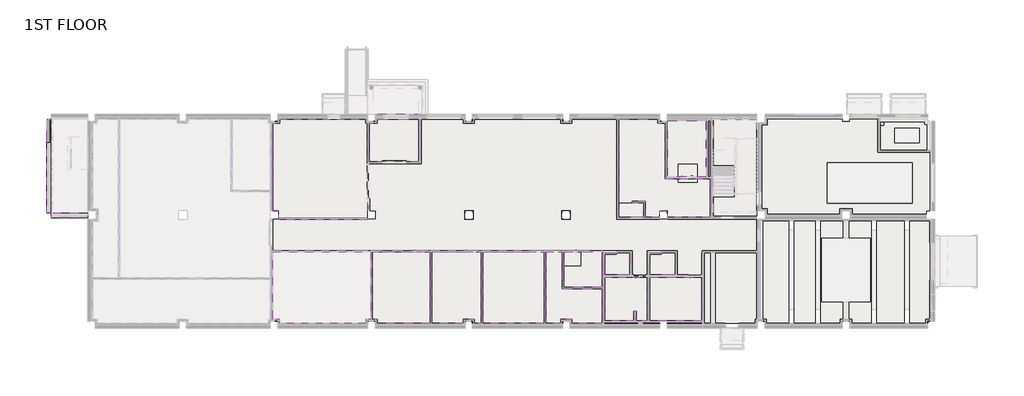
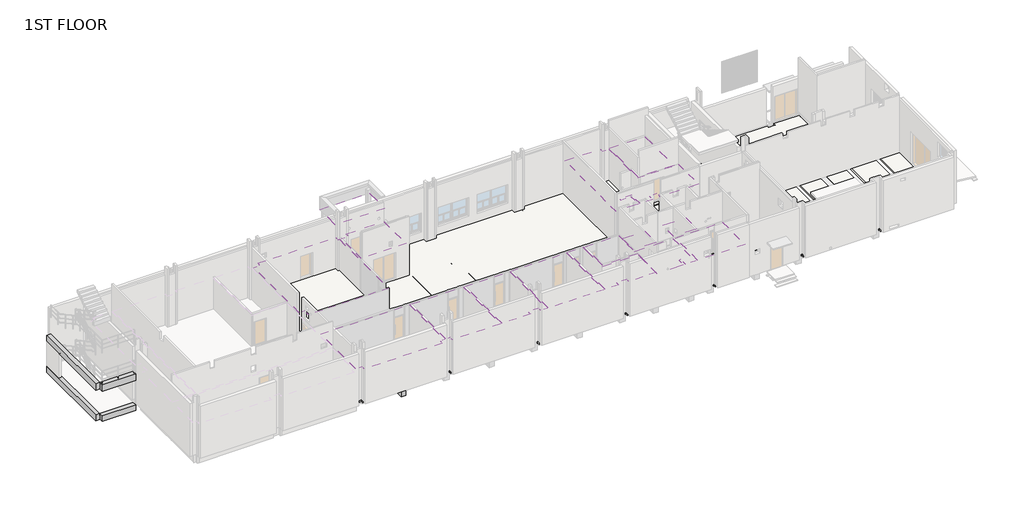
# One storey, part 8 of 15: 26 slabs, 15 coverings, 5 beams.
# Revit data of these elements (continued)
# Type "H_CE_AR_B09_2L Gypsum Board_T Bar_9T_C4" (continued)
#   Layers, outside or top first: 9.5 mm "00_Finish_Gypsum Board" (function 4); 9.5 mm "00_Finish_Gypsum Board" (function 4)
# Type "H_CE_AR_B09_Aluminum Spandrel_M Bar_0.8T_C9"
#   built-in parameter 1002203 = 1 (stored number, unit not read)
#   built-in parameter 1002202 = 1 (stored number, unit not read)
#   Layers, outside or top first: 0.8 mm "00.Ceiling_Aluminum Spandrel" (function 4)
# Type "H_CE_AR_B09_SMC Ceiling_T Bar_300x300x0.8T_C6"
#   built-in parameter 1002203 = 1 (stored number, unit not read)
#   built-in parameter 1002202 = 1 (stored number, unit not read)
#   Layers, outside or top first: 0.8 mm "00.Ceiling_SMC" (function 4)
# Type "H_CE_AR_B09_Souns Absorbing Soft Fiber Board_T Bar_600x600x9T_C5"
#   built-in parameter 1002203 = 1 (stored number, unit not read)
#   built-in parameter 1002202 = 1 (stored number, unit not read)
#   Layers, outside or top first: 9 mm "00.Ceiling_Sound Absorbing Soft Fiber Board" (function 4)
# Type "H_CE_AR_B09_Stainless Hairline Finish_3T"
#   built-in parameter 1002203 = 1 (stored number, unit not read)
#   built-in parameter 1002202 = 1 (stored number, unit not read)
#   Layers, outside or top first: 3 mm "00.Finish_Stainless Hairline" (function 4)
# Type "H_FL_AR_S17_RC Slab_T150_1S1"
#   Keynote = ""
#   Type Comments = "CV-AG"
#   Description = ""
#   H_Rebar Ratio = 0.1
#   Function = 1
#   Layers, outside or top first: 150 mm "Concrete_f'c=28MPa(Cylender)" (function 1)
# Type "H_FL_AR_S17_RC Slab_T150_GS1"
#   Keynote = ""
#   Type Comments = "CV-AG"
#   Description = ""
#   H_Rebar Ratio = 0.1
#   Function = 1
#   Layers, outside or top first: 150 mm "Concrete_f'c=28MPa(Cylender)" (function 1)
# Type "H_FL_AR_S17_RC Slab_T200_SS1"
#   Keynote = ""
#   Type Comments = "CV-AG"
#   Description = ""
#   H_Rebar Ratio = 0.1
#   Function = 1
#   Layers, outside or top first: 200 mm "Concrete_f'c=28MPa(Cylender)" (function 1)
# Type "H_FL_AR_B07_Wood Tile_600x600xT3_F8"
#   Keynote = ""
#   Type Comments = "Finish"
#   Description = ""
#   Function = 1
#   Layers, outside or top first: 3 mm "00_Finish_Wood Tile" (function 4); 27 mm "00_Concrete_Cement Mortar" (function 1)
# Type "H_FL_AR_B07_Deco Tile_600x600xT3"
#   Keynote = ""
#   Type Comments = "Finish"
#   Description = ""
#   Function = 1
#   Layers, outside or top first: 3 mm "00_Finish_Deco Tile" (function 4); 27 mm "00_Concrete_Cement Mortar" (function 1)
# Type "H_FL_AR_B07_Polishing Tile_600x600xT3"
#   Keynote = ""
#   Type Comments = "Finish"
#   Description = ""
#   Function = 1
#   Layers, outside or top first: 3 mm "00_Finish_Polishing Tile" (function 4); 27 mm "00_Concrete_Cement Mortar" (function 1)
# Type "H_FL_AR_B07_Capet Tile_600x600xT3"
#   Keynote = ""
#   Type Comments = "Finish"
#   Description = ""
#   Function = 1
#   Layers, outside or top first: 3 mm "00_Finish_Carpet Tile" (function 4); 27 mm "00_Concrete_Cement Mortar" (function 1)
# Type "H_FL_AR_B07_Wood Tile_600x600xT110_F8"
#   Keynote = ""
#   Type Comments = "Finish"
#   Description = ""
#   Function = 1
#   Layers, outside or top first: 3 mm "00_Finish_Wood Tile" (function 4); 107 mm "00_Concrete_Cement Mortar" (function 1)
# Type "H_FL_AR_B07_Non-Slip Ceramic Tile_L Waterproof_300x300xT4"
#   Keynote = ""
#   Type Comments = "Finish"
#   Description = ""
#   Function = 0
#   Layers, outside or top first: 4 mm "00_Finish_Ceramic Tile" (function 4); 96 mm "00_Concrete_Cement Mortar" (function 1)
# Type "H_FL_AR_B07_Granite Tile_150x150xT30"
#   Keynote = ""
#   Type Comments = "Finish"
#   Description = ""
#   Function = 0
#   Layers, outside or top first: 30 mm "00_Stone_Granite" (function 4); 60 mm "00_Concrete_Cement Mortar" (function 1)
# Type "H_FL_AR_B07_Granite Tile_150x150xT30(Mortar_T170)"
#   Keynote = ""
#   Type Comments = "Finish"
#   Description = ""
#   Function = 0
#   Layers, outside or top first: 30 mm "00_Stone_Granite" (function 4); 170 mm "00_Concrete_Cement Mortar" (function 1)
# Type "H_FL_AR_S17_RC Slab_T300"
#   Keynote = ""
#   Type Comments = "CV-AG"
#   Description = ""
#   H_Rebar Ratio = 0.12
#   Function = 1
#   Layers, outside or top first: 300 mm "Concrete_f'c=28MPa(Cylender)" (function 1)
# Element 1 (IfcBeam, "RC Beam_Rectangular : H_SB_AR S16_TG-UG_450x800_1B1A")
#   Comments = ""
#   hec_material3 = none
#   hec_material2 = none
#   hec_material1 = none
#   Structural Material = Concrete_f'c=28MPa(Cylender)
#   Phase Created = New Construction
#   Materials on its faces: "Concrete_f'c=28MPa(Cylender)"
# Element 2 (IfcBeam, "RC Beam_Rectangular : H_SB_AR S16_RC Beam-AG_400x530_SG1A")
#   Comments = ""
#   hec_material3 = none
#   hec_material2 = none
#   hec_material1 = none
#   Structural Material = Concrete_f'c=28MPa(Cylender)
#   Phase Created = New Construction
#   Materials on its faces: "Concrete_f'c=28MPa(Cylender)"
# Element 3 (IfcBeam, "RC Beam_Rectangular : H_SB_AR S16_RC Beam-AG_400x600_SG2")
#   Comments = ""
#   hec_material3 = none
#   hec_material2 = none
#   hec_material1 = none
#   Structural Material = Concrete_f'c=28MPa(Cylender)
#   Phase Created = New Construction
#   Materials on its faces: "Concrete_f'c=28MPa(Cylender)"
# Element 4 (IfcBeam, "RC Beam_Rectangular : H_SB_AR S16_RC Beam-AG_400x600_SWG2")
#   Comments = ""
#   hec_material3 = none
#   hec_material2 = none
#   hec_material1 = none
#   Structural Material = Concrete_f'c=28MPa(Cylender)
#   Phase Created = New Construction
#   Materials on its faces: "Concrete_f'c=28MPa(Cylender)"
# Element 5 (IfcBeam, "RC Beam_Rectangular : H_SB_AR S16_RC Beam-AG_400x600_SG1")
#   Comments = ""
#   hec_material3 = none
#   hec_material2 = none
#   hec_material1 = none
#   Structural Material = Concrete_f'c=28MPa(Cylender)
#   Phase Created = New Construction
#   Materials on its faces: "Concrete_f'c=28MPa(Cylender)"
# Elements 6, 10, 11, 13 (IfcCovering, "H_CE_AR_B09_2L Gypsum Board_T Bar_9T_C4")
#   Height Offset From Level = 3030 mm
#   Phase Created = New Construction
#   Materials on its faces: "00_Finish_Gypsum Board"
# Element 7 (IfcCovering, "H_CE_AR_B09_Aluminum Spandrel_M Bar_0.8T_C9")
#   Height Offset From Level = 3030 mm
#   Phase Created = New Construction
#   Materials on its faces: "00.Ceiling_Aluminum Spandrel"
# Element 8 (IfcCovering, "H_CE_AR_B09_2L Gypsum Board_T Bar_9T_C4")
#   Height Offset From Level = 3110 mm
#   Phase Created = New Construction
#   Materials on its faces: "00_Finish_Gypsum Board"
# Element 9 (IfcCovering, "H_CE_AR_B09_SMC Ceiling_T Bar_300x300x0.8T_C6")
#   Height Offset From Level = 3000 mm
#   Phase Created = New Construction
#   Materials on its faces: "00.Ceiling_SMC"
# Elements 12, 14, 15 (IfcCovering, "H_CE_AR_B09_Souns Absorbing Soft Fiber Board_T Bar_600x600x9T_C5")
#   Height Offset From Level = 3030 mm
#   Phase Created = New Construction
#   Materials on its faces: "00.Ceiling_Sound Absorbing Soft Fiber Board"
# Elements 16, 17, 18, 19 (IfcCovering, "H_CE_AR_B09_2L Gypsum Board_T Bar_9T_C4")
#   Height Offset From Level = 2700 mm
#   Phase Created = New Construction
#   Materials on its faces: "00_Finish_Gypsum Board"
# Element 20 (IfcCovering, "H_CE_AR_B09_Stainless Hairline Finish_3T")
#   Height Offset From Level = 3900 mm
#   Phase Created = New Construction
#   Materials on its faces: "00.Finish_Stainless Hairline"
# Element 21 (IfcSlab, "H_FL_AR_S17_RC Slab_T150_1S1")
#   Comments = ""
#   TMP_Element Name = "SS2"
#   Height Offset From Level = 0 mm
#   built-in parameter 1001954 = 1
#   Phase Created = New Construction
#   Materials on its faces: "Concrete_f'c=28MPa(Cylender)"
# Element 22 (IfcSlab, "H_FL_AR_S17_RC Slab_T150_1S1")
#   Comments = ""
#   TMP_Element Name = "SS2"
#   Height Offset From Level = -100 mm
#   built-in parameter 1001954 = 1
#   Phase Created = New Construction
#   Materials on its faces: "Concrete_f'c=28MPa(Cylender)"
# Element 23 (IfcSlab, "H_FL_AR_S17_RC Slab_T150_GS1")
#   Comments = ""
#   TMP_Element Name = "SS2"
#   built-in parameter 1001955 = 3.14159 (stored number, unit not read)
#   Height Offset From Level = 0 mm
#   built-in parameter 1001954 = 1
#   Phase Created = New Construction
#   Materials on its faces: "Concrete_f'c=28MPa(Cylender)"
# Element 24 (IfcSlab, "H_FL_AR_S17_RC Slab_T150_1S1")
#   Comments = ""
#   TMP_Element Name = "SS2"
#   built-in parameter 1001955 = 3.14159 (stored number, unit not read)
#   Height Offset From Level = -100 mm
#   built-in parameter 1001954 = 1
#   Phase Created = New Construction
#   Materials on its faces: "Concrete_f'c=28MPa(Cylender)"
# Element 25 (IfcSlab, "H_FL_AR_S17_RC Slab_T200_SS1")
#   Comments = ""
#   TMP_Element Name = "SS2"
#   Height Offset From Level = 0 mm
#   built-in parameter 1001954 = 1
#   Phase Created = New Construction
#   Materials on its faces: "Concrete_f'c=28MPa(Cylender)"
# Element 26 (IfcSlab, "H_FL_AR_S17_RC Slab_T150_GS1")
#   Comments = ""
#   TMP_Element Name = "SS2"
#   Height Offset From Level = 0 mm
#   built-in parameter 1001954 = 1
#   Phase Created = New Construction
#   Materials on its faces: "Concrete_f'c=28MPa(Cylender)"
# Elements 27, 43 (IfcSlab, "H_FL_AR_B07_Wood Tile_600x600xT3_F8")
#   Height Offset From Level = 30 mm
#   Phase Created = New Construction
#   Materials on its faces: "00_Concrete_Cement Mortar", "00_Finish_Wood Tile"
# Elements 28, 31, 40, 42 (IfcSlab, "H_FL_AR_B07_Deco Tile_600x600xT3")
#   Height Offset From Level = 30 mm
#   Phase Created = New Construction
#   Materials on its faces: "00_Concrete_Cement Mortar", "00_Finish_Deco Tile"
# Element 29 (IfcSlab, "H_FL_AR_B07_Polishing Tile_600x600xT3")
#   built-in parameter 1001955 = 1.5708 (stored number, unit not read)
#   Height Offset From Level = 30 mm
#   Phase Created = New Construction
#   Materials on its faces: "00_Concrete_Cement Mortar", "00_Finish_Polishing Tile"
# Element 30 (IfcSlab, "H_FL_AR_B07_Wood Tile_600x600xT3_F8")
#   built-in parameter 1001955 = 1.5708 (stored number, unit not read)
#   Height Offset From Level = 30 mm
#   Phase Created = New Construction
#   Materials on its faces: "00_Concrete_Cement Mortar", "00_Finish_Wood Tile"
# Element 32 (IfcSlab, "H_FL_AR_B07_Capet Tile_600x600xT3")
#   Height Offset From Level = 30 mm
#   Phase Created = New Construction
#   Materials on its faces: "00_Concrete_Cement Mortar", "00_Finish_Carpet Tile"
# Element 33 (IfcSlab, "H_FL_AR_B07_Deco Tile_600x600xT3")
#   built-in parameter 1001955 = 1.5708 (stored number, unit not read)
#   Height Offset From Level = 30 mm
#   Phase Created = New Construction
#   Materials on its faces: "00_Concrete_Cement Mortar", "00_Finish_Deco Tile"
# Element 34 (IfcSlab, "H_FL_AR_B07_Wood Tile_600x600xT110_F8")
#   Height Offset From Level = 110 mm
#   Phase Created = New Construction
#   Materials on its faces: "00_Concrete_Cement Mortar", "00_Finish_Wood Tile"
# Elements 35, 36, 37, 38, 41 (IfcSlab, "H_FL_AR_B07_Non-Slip Ceramic Tile_L Waterproof_300x300xT4")
#   Height Offset From Level = 0 mm
#   Phase Created = New Construction
#   Materials on its faces: "00_Concrete_Cement Mortar", "00_Finish_Ceramic Tile"
# Element 39 (IfcSlab, "H_FL_AR_B07_Wood Tile_600x600xT110_F8")
#   built-in parameter 1001955 = 1.5708 (stored number, unit not read)
#   Height Offset From Level = 110 mm
#   Phase Created = New Construction
#   Materials on its faces: "00_Concrete_Cement Mortar", "00_Finish_Wood Tile"
# Element 44 (IfcSlab, "H_FL_AR_B07_Granite Tile_150x150xT30")
#   Height Offset From Level = 200 mm
#   Phase Created = New Construction
#   Materials on its faces: "00_Concrete_Cement Mortar", "00_Stone_Granite"
# Element 45 (IfcSlab, "H_FL_AR_B07_Granite Tile_150x150xT30(Mortar_T170)")
#   Height Offset From Level = 200 mm
#   Phase Created = New Construction
#   Materials on its faces: "00_Concrete_Cement Mortar", "00_Stone_Granite"
# Element 46 (IfcSlab, "H_FL_AR_S17_RC Slab_T300")
#   Comments = ""
#   TMP_Element Name = "SS2"
#   Height Offset From Level = -150 mm
#   built-in parameter 1001954 = 1
#   Phase Created = New Construction
#   Materials on its faces: "Concrete_f'c=28MPa(Cylender)"
# Materials
#   "00_Finish_Gypsum Board": class "Finish", colour RGB 171 170 168, transparency 0, Description = "Gypsum Board", Cost = 0, Image = Finishes.Gypsum Board.Painted.White.jpg
#   "00.Ceiling_Aluminum Spandrel": class "Generic", colour RGB 253 254 255, transparency 0, Description = "Acoustic ceiling tile", Cost = 0
#   "00.Ceiling_SMC": class "Generic", colour RGB 237 237 236, transparency 0, Description = "Acoustic ceiling tile", Cost = 0
#   "00.Ceiling_Sound Absorbing Soft Fiber Board": class "Generic", colour RGB 237 237 236, transparency 0, Description = "Acoustic ceiling tile", Cost = 0
#   "00.Finish_Stainless Hairline": class "Generic", colour RGB 149 149 149, transparency 0, Description = "Acoustic ceiling tile", Cost = 0
#   "Concrete_f'c=28MPa(Cylender)": class "Concrete", colour RGB 176 176 176, transparency 0, Description = "Reinf. Conc.", Cost = 0, Image = Concrete.Cast-In-Place.Flat.Polished.Grey.jpg
#   "00_Finish_Wood Tile": class "Finish", colour RGB 233 219 207, transparency 0, Description = "Ceramic Tile", Cost = 0
#   "00_Concrete_Cement Mortar": class "Concrete", colour RGB 183 186 184, transparency 0, Description = "Cement Mortar", Cost = 0, Image = Concrete.Cast-In-Place.Flat.Broom.Grey.jpg
#   "00_Finish_Deco Tile": class "Finish", colour RGB 245 245 245, transparency 0, Description = "Ceramic Tile", Cost = 0
#   "00_Finish_Polishing Tile": class "Finish", colour RGB 245 245 245, transparency 0, Description = "Ceramic Tile", Cost = 0
#   "00_Finish_Carpet Tile": class "Finish", colour RGB 68 67 66, transparency 0, Description = "Carpet", Cost = 0
#   "00_Finish_Ceramic Tile": class "Finish", colour RGB 245 245 245, transparency 0, Description = "Ceramic Tile", Cost = 0, Image = none
#   "00_Stone_Granite": class "Stone", colour RGB 99 103 98, transparency 0, Description = "Granite", Cost = 0, Image = Masonry.Stone.Granite.Square.Stacked.Polished.Black-White.jpg
# Room at (66747.5, -1477.5) mm, phase "New Construction", upper level "1ST FLOOR", upper offset 5800 mm, lower offset 0 mm
#   Comments = ""
#   Occupancy = "1"
#   Number = "124"
#   Name = "F.O TANK ROOM"
#   H_Room H or CH = 5800 mm
# Room at (48912.5, -2537.5) mm, phase "New Construction", upper level "1ST FLOOR", upper offset 5800 mm, lower offset 0 mm
#   Comments = ""
#   Occupancy = "1"
#   Number = "109"
#   Name = "SHOWER ROOM"
#   H_Room H or CH = 3000 mm
# Room at (61920.25, -12686.25) mm, phase "New Construction", upper level "1ST FLOOR", upper offset 5800 mm, lower offset 0 mm
#   Comments = ""
#   Occupancy = "1"
#   Number = "125"
#   Name = "HVAC ROOM"
#   H_Room H or CH = 5800 mm
# Room at (24871.5, -1826.5) mm, phase "New Construction", upper level "1ST FLOOR", upper offset 5800 mm, lower offset 0 mm
#   Comments = ""
#   Occupancy = "1"
#   Number = "105"
#   Name = "AIR LOCK"
#   H_Room H or CH = 3000 mm
# Room at (52496.5, -14023.5) mm, phase "New Construction", upper level "1ST FLOOR", upper offset 5800 mm, lower offset 0 mm
#   Comments = ""
#   Occupancy = "1"
#   Number = "122"
#   Name = "CYLINDER ROOM"
#   H_Room H or CH = 3000 mm
# Room at (43200, -12000) mm, phase "New Construction", upper level "1ST FLOOR", upper offset 5800 mm, lower offset 0 mm
#   Comments = ""
#   Occupancy = "1"
#   Number = "118"
#   Name = "DISABLED TOLET(M)"
#   H_Room H or CH = 2700 mm
# Room at (43900, -14887.5) mm, phase "New Construction", upper level "1ST FLOOR", upper offset 5800 mm, lower offset 0 mm
#   Comments = ""
#   Occupancy = "1"
#   Number = "120"
#   Name = "TOILET(M)"
#   H_Room H or CH = 2700 mm
# Room at (46900, -12000) mm, phase "New Construction", upper level "1ST FLOOR", upper offset 5800 mm, lower offset 0 mm
#   Comments = ""
#   Occupancy = "1"
#   Number = "119"
#   Name = "DISABLED TOILET(W)"
#   H_Room H or CH = 2700 mm
# Room at (48000, -14887.5) mm, phase "New Construction", upper level "1ST FLOOR", upper offset 5800 mm, lower offset 0 mm
#   Comments = ""
#   Occupancy = "1"
#   Number = "121"
#   Name = "TOILET(W)"
#   H_Room H or CH = 2700 mm
# Room at (47084, -5635.02) mm, phase "New Construction", upper level "1ST FLOOR", upper offset 5800 mm, lower offset 0 mm
#   Comments = ""
#   Occupancy = "1"
#   Number = "108"
#   Name = "LOCKER ROOM"
#   H_Room H or CH = 3000 mm
# Room at (34768, -8500) mm, phase "New Construction", upper level "1ST FLOOR", upper offset 5800 mm, lower offset 0 mm
#   Comments = ""
#   Occupancy = "1"
#   Number = "111"
#   Name = "CORRIDOR"
#   H_Room H or CH = 5800 mm
# Room at (52862.5, -4131) mm, phase "New Construction", upper level "1ST FLOOR", upper offset 5800 mm, lower offset 0 mm
#   Comments = ""
#   Occupancy = "1"
#   Number = "110"
#   Name = "STAIRCASE"
#   H_Room H or CH = 5800 mm
# Room at (62081, -3919) mm, phase "New Construction", upper level "1ST FLOOR", upper offset 9300 mm, lower offset 0 mm
#   Comments = ""
#   Number = "123"
#   Name = "EDG ROOM"
#   H_Room H or CH = 9200 mm
# Room at (44419.201, -7539.972) mm, phase "New Construction", upper level "1ST FLOOR", upper offset 5800 mm, lower offset 0 mm
#   Comments = ""
#   Occupancy = "1"
#   Number = "151"
#   Name = "LOCKER ENTRANCE"
#   H_Room H or CH = 3000 mm
# Room at (33678.344, -3773.505) mm, phase "New Construction", upper level "1ST FLOOR", upper offset 5800 mm, lower offset 0 mm
#   Comments = ""
#   Occupancy = "1"
#   Number = "107"
#   Name = "OFFICE ROOM"
#   H_Room H or CH = 5800 mm
# Room at (40496.214, -12367.394) mm, phase "New Construction", upper level "1ST FLOOR", upper offset 5800 mm, lower offset 0 mm
#   Comments = ""
#   Occupancy = "1"
#   Number = "116"
#   Name = "MAMA'S REST ROOM"
#   H_Room H or CH = 3000 mm
# Room at (39361.919, -14919.559) mm, phase "New Construction", upper level "1ST FLOOR", upper offset 5800 mm, lower offset 0 mm
#   Comments = ""
#   Occupancy = "1"
#   Number = "117"
#   Name = "STORAGE"
#   H_Room H or CH = 3000 mm
# Room at (34862.546, -13898.693) mm, phase "New Construction", upper level "1ST FLOOR", upper offset 5800 mm, lower offset 0 mm
#   Comments = ""
#   Occupancy = "1"
#   Number = "115"
#   Name = "PRESIDENT ROOM"
#   H_Room H or CH = 3000 mm
# Room at (30211.935, -13917.598) mm, phase "New Construction", upper level "1ST FLOOR", upper offset 5800 mm, lower offset 0 mm
#   Comments = ""
#   Occupancy = "1"
#   Number = "114"
#   Name = "PARTNER'S OFFICE"
#   H_Room H or CH = 3000 mm
# Room at (25315.559, -14049.933) mm, phase "New Construction", upper level "1ST FLOOR", upper offset 5800 mm, lower offset 0 mm
#   Comments = ""
#   Occupancy = "1"
#   Number = "113"
#   Name = "REST ROOM"
#   H_Room H or CH = 3000 mm
# Room at (19265.983, -13936.503) mm, phase "New Construction", upper level "1ST FLOOR", upper offset 5800 mm, lower offset 0 mm
#   Comments = ""
#   Occupancy = "1"
#   Number = "112"
#   Name = "CONFERENCE ROOM"
#   H_Room H or CH = 3000 mm
# Room at (18995.787, -4264.529) mm, phase "New Construction", upper level "1ST FLOOR", upper offset 5800 mm, lower offset 0 mm
#   Comments = ""
#   Occupancy = "1"
#   Number = "104"
#   Name = "CANTEEN"
#   H_Room H or CH = 3000 mm
# Room at (12951.563, -3235.471) mm, phase "New Construction", upper level "1ST FLOOR", upper offset 5800 mm, lower offset 0 mm
#   Comments = ""
#   Occupancy = "1"
#   Number = "102"
#   Name = "MEETING ROOM"
#   H_Room H or CH = 3000 mm
# Room at (8524.954, -7021.7) mm, phase "New Construction", upper level "1ST FLOOR", upper offset 5800 mm, lower offset 0 mm
#   Comments = ""
#   Occupancy = "1"
#   Number = "101"
#   Name = "CENTRAL CONTROL ROOM"
#   H_Room H or CH = 3000 mm
# Room at (1443.913, -5932.309) mm, phase "New Construction", upper level "1ST FLOOR", upper offset 5800 mm, lower offset 0 mm
#   Comments = ""
#   Occupancy = "1"
#   Number = "152"
#   Name = "CCR SIDE"
#   H_Room H or CH = 3000 mm
# Room at (5610.834, -15410.011) mm, phase "New Construction", upper level "1ST FLOOR", upper offset 5800 mm, lower offset 0 mm
#   Comments = ""
#   Occupancy = "1"
#   Number = "103"
#   Name = "ENGINEERING ROOM"
#   H_Room H or CH = 3000 mm
